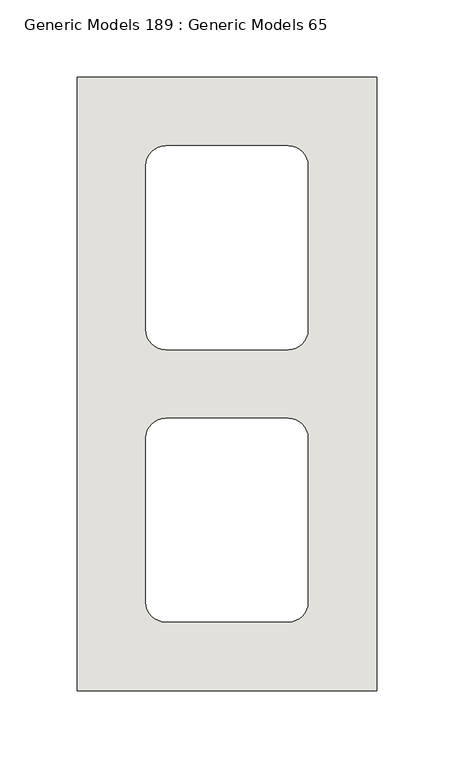
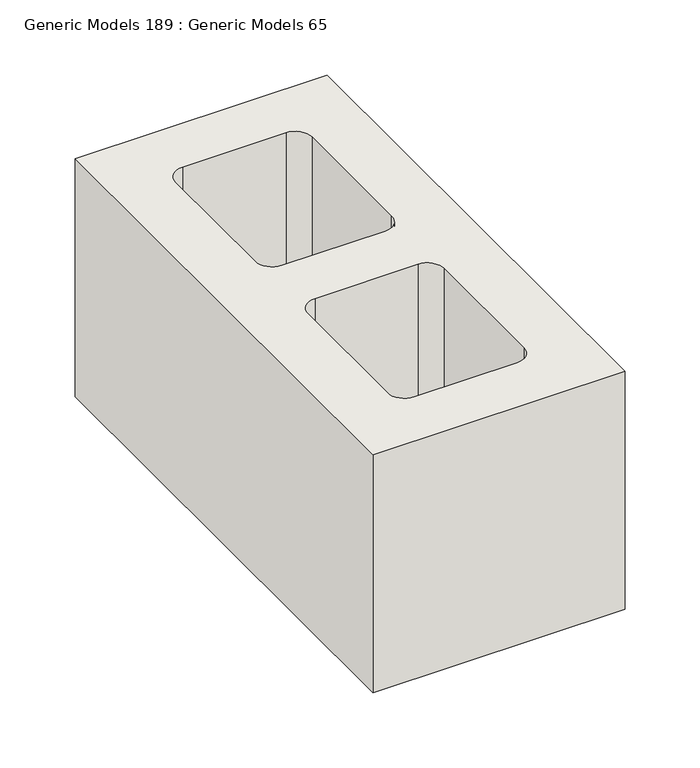
"""IFC4 building model written with IfcOpenShell, lengths in millimetres: wall geometry, Generic Models 189 : Generic Models 65."""

from ifc_helpers import new_model, si_unit, point, frame, frame_2d, origin, place, context, project, spatial, polyline, circle_curve, trimmed, segment, composite_curve, outline, extrude, source, transform, mapped, element, save


def generic_models_189_generic_models_65_b86c8691(model_context):
    return source(origin(), model_context, "Body", "SweptSolid", [
        extrude(outline(polyline([(375199.1901825, 292.1), (375005.5151825, 292.1), (375005.5151825, 688.975), (375199.1901825, 688.975), (375199.1901825, 292.1)]), holes=[composite_curve([segment(polyline([(375154.7401825, 525.4625), (375154.7401825, 631.825)]), True, "CONTINUOUS"), segment(trimmed(circle_curve(frame_2d((375142.0401825, 631.825)), 12.7), [point((375154.7401825, 631.825))], [point((375142.0401825, 644.525))], True, "CARTESIAN"), True, "CONTINUOUS"), segment(polyline([(375142.0401825, 644.525), (375062.6651825, 644.525)]), True, "CONTINUOUS"), segment(trimmed(circle_curve(frame_2d((375062.6651825, 631.825)), 12.7), [point((375062.6651825, 644.525))], [point((375049.9651825, 631.825))], True, "CARTESIAN"), True, "CONTINUOUS"), segment(polyline([(375049.9651825, 631.825), (375049.9651825, 525.4625)]), True, "CONTINUOUS"), segment(trimmed(circle_curve(frame_2d((375062.6651825, 525.4625)), 12.7), [point((375049.9651825, 525.4625))], [point((375062.6651825, 512.7625))], True, "CARTESIAN"), True, "CONTINUOUS"), segment(polyline([(375062.6651825, 512.7625), (375142.0401825, 512.7625)]), True, "CONTINUOUS"), segment(trimmed(circle_curve(frame_2d((375142.0401825, 525.4625)), 12.7), [point((375142.0401825, 512.7625))], [point((375154.7401825, 525.4625))], True, "CARTESIAN"), True, "CONTINUOUS")], self_intersect=False), composite_curve([segment(polyline([(375049.9651825, 455.6125), (375049.9651825, 349.25)]), True, "CONTINUOUS"), segment(trimmed(circle_curve(frame_2d((375062.6651825, 349.25)), 12.7), [point((375049.9651825, 349.25))], [point((375062.6651825, 336.55))], True, "CARTESIAN"), True, "CONTINUOUS"), segment(polyline([(375062.6651825, 336.55), (375142.0401825, 336.55)]), True, "CONTINUOUS"), segment(trimmed(circle_curve(frame_2d((375142.0401825, 349.25)), 12.7), [point((375142.0401825, 336.55))], [point((375154.7401825, 349.25))], True, "CARTESIAN"), True, "CONTINUOUS"), segment(polyline([(375154.7401825, 349.25), (375154.7401825, 455.6125)]), True, "CONTINUOUS"), segment(trimmed(circle_curve(frame_2d((375142.0401825, 455.6125)), 12.7), [point((375154.7401825, 455.6125))], [point((375142.0401825, 468.3125))], True, "CARTESIAN"), True, "CONTINUOUS"), segment(polyline([(375142.0401825, 468.3125), (375062.6651825, 468.3125)]), True, "CONTINUOUS"), segment(trimmed(circle_curve(frame_2d((375062.6651825, 455.6125)), 12.7), [point((375062.6651825, 468.3125))], [point((375049.9651825, 455.6125))], True, "CARTESIAN"), True, "CONTINUOUS")], self_intersect=False)]), frame((0.0, 0.0, 2193.3712588), z_axis=(0.0, 0.0, 1.0), x_axis=(1.0, 0.0, 0.0)), (0.0, 0.0, 1.0), 193.675),
    ])


if __name__ == "__main__":
    model = new_model("IFC4")
    model_context = context("Model", 3, world=origin())
    ifc_project = project(units=[si_unit("LENGTHUNIT", "METRE", prefix="MILLI")], contexts=[model_context])
    site = spatial("IfcSite", under=ifc_project)
    building = spatial("IfcBuilding", under=site)
    placement = place(None, origin())
    generic_models_189_generic_models_65_shape = generic_models_189_generic_models_65_b86c8691(model_context)
    element("IfcWall", 1, ObjectType="Generic Models 189 : Generic Models 65", at=placement, inside=building, context=model_context, shape_type="MappedRepresentation", body=[
        mapped(generic_models_189_generic_models_65_shape, transform((0.0, 0.0, 0.0), x_axis=(1.0, 0.0, 0.0), y_axis=(0.0, 1.0, 0.0), z_axis=(0.0, 0.0, 1.0))),
    ])
    save(model, "model.ifc")

# Revit data of these elements
# Element 1 (IfcWall, "Generic Models 189 : Generic Models 65")
#   Materials on its faces: "CMU (SEE 'WALL TAG' FOR SIZE)"
# Materials
#   "CMU (SEE 'WALL TAG' FOR SIZE)": class "Masonry", colour RGB 203 203 199, transparency 0, Description = "Concrete masonry units", Cost = 0
